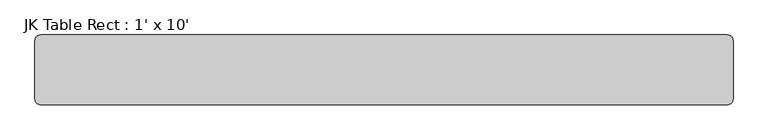
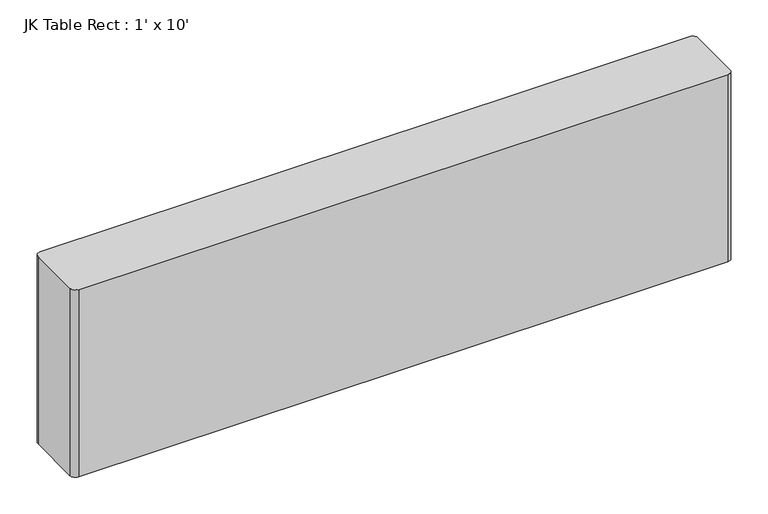
"""IFC4 building model written with IfcOpenShell, lengths in millimetres: furniture geometry, JK Table Rect : 1' x 10'."""

import ifcopenshell
import ifcopenshell.guid

model = None  # the IFC model being written
_history = None  # IfcOwnerHistory: only IFC2X3 demands one
_inside = {}  # id of a spatial element -> (the spatial element, [elements in it])
_under = {}  # id of a project, library or spatial element -> (it, [spatial elements below it])
_declared = {}  # id of a project -> (the project, [libraries it declares])
_typed = {}  # id of a type object -> (the type object, [elements of that type])
_made_of = {}  # id of a material, layer set ... -> (it, [elements and type objects made of it])


def new_model(schema):
    """Start an empty IFC model of exactly this schema.

    Asked for "IFC4X3", IfcOpenShell would pick the latest addendum, in which some entities
    have other attributes; the version numbers below select the first issue.
    IFC2X3 requires an IfcOwnerHistory on every rooted entity: one is made here for all.
    """
    global model, _history
    if schema == "IFC4X3":
        model = ifcopenshell.file(schema_version=(4, 3, 0, 0))
    else:
        model = ifcopenshell.file(schema=schema)
    _inside.clear()
    _under.clear()
    _declared.clear()
    _typed.clear()
    _made_of.clear()
    _history = None
    if model.schema == "IFC2X3":
        org = make("IfcOrganization", Name="unknown")
        user = make(
            "IfcPersonAndOrganization",
            ThePerson=make("IfcPerson", FamilyName="unknown"),
            TheOrganization=org,
        )
        app = make(
            "IfcApplication",
            ApplicationDeveloper=org,
            Version="unknown",
            ApplicationFullName="unknown",
            ApplicationIdentifier="unknown",
        )
        _history = make(
            "IfcOwnerHistory",
            OwningUser=user,
            OwningApplication=app,
            ChangeAction="ADDED",
            CreationDate=0,
        )
    return model


def make(cls, **values):
    """One entity of the class cls with the attributes given. An attribute that is None is left unset."""
    return model.create_entity(
        cls, **{name: value for name, value in values.items() if value is not None}
    )


def rooted(cls, **values):
    """An entity with a GlobalId (a new one), such as an element, a storey or a relation."""
    return make(cls, GlobalId=ifcopenshell.guid.new(), OwnerHistory=_history, **values)


def si_unit(unit_type, name, prefix=None):
    """IfcSIUnit, for example si_unit("LENGTHUNIT", "METRE", prefix="MILLI")."""
    return make("IfcSIUnit", UnitType=unit_type, Prefix=prefix, Name=name)


def assignment(units):
    """IfcUnitAssignment: the units of a project."""
    return None if units is None else make("IfcUnitAssignment", Units=units)


def point(xyz):
    """IfcCartesianPoint."""
    return None if xyz is None else make("IfcCartesianPoint", Coordinates=xyz)


def direction(xyz):
    """IfcDirection."""
    return None if xyz is None else make("IfcDirection", DirectionRatios=xyz)


def frame(location, z_axis=None, x_axis=None):
    """IfcAxis2Placement3D, a coordinate frame: its origin and axes. An axis left out is left unset."""
    return make(
        "IfcAxis2Placement3D",
        Location=point(location),
        Axis=direction(z_axis),
        RefDirection=direction(x_axis),
    )


def frame_2d(location, x_axis=None):
    """IfcAxis2Placement2D, a coordinate frame in the plane: its origin and x axis."""
    return make(
        "IfcAxis2Placement2D", Location=point(location), RefDirection=direction(x_axis)
    )


def origin():
    """The frame at (0, 0, 0) with its axes left unset."""
    return frame((0.0, 0.0, 0.0))


def origin_with_axes():
    """The frame at (0, 0, 0) with the z axis (0, 0, 1) and the x axis (1, 0, 0) written out."""
    return frame((0.0, 0.0, 0.0), z_axis=(0.0, 0.0, 1.0), x_axis=(1.0, 0.0, 0.0))


def place(relative_to, where):
    """IfcLocalPlacement: puts the frame where relative to a parent placement (None: the world)."""
    return make(
        "IfcLocalPlacement", PlacementRelTo=relative_to, RelativePlacement=where
    )


def context(
    kind, dimensions, precision=None, world=None, true_north=None, identifier=None
):
    """IfcGeometricRepresentationContext, for example the 3D "Model" context."""
    return make(
        "IfcGeometricRepresentationContext",
        ContextIdentifier=identifier,
        ContextType=kind,
        CoordinateSpaceDimension=dimensions,
        Precision=precision,
        WorldCoordinateSystem=world,
        TrueNorth=true_north,
    )


def project(units=None, contexts=None):
    """IfcProject with its units and contexts."""
    return rooted(
        "IfcProject",
        Name="project",
        RepresentationContexts=contexts,
        UnitsInContext=assignment(units),
    )


def spatial(cls, under=None, at=None, **own):
    """A site, building, storey or space (cls), placed at a placement, below another one or the project."""
    s = rooted(cls, ObjectPlacement=at, **own)
    if under is not None:
        _under.setdefault(under.id(), (under, []))[1].append(s)
    return s


def polyline(points):
    """IfcPolyline through the points."""
    return make("IfcPolyline", Points=[point(p) for p in points])


def circle_curve(where, radius):
    """IfcCircle in the frame where."""
    return make("IfcCircle", Position=where, Radius=radius)


def trimmed(basis, trim1, trim2, sense, master):
    """IfcTrimmedCurve: the piece of a basis curve between two trims."""
    return make(
        "IfcTrimmedCurve",
        BasisCurve=basis,
        Trim1=trim1,
        Trim2=trim2,
        SenseAgreement=sense,
        MasterRepresentation=master,
    )


def segment(curve, same_sense, transition):
    """IfcCompositeCurveSegment."""
    return make(
        "IfcCompositeCurveSegment",
        Transition=transition,
        SameSense=same_sense,
        ParentCurve=curve,
    )


def composite_curve(segments, self_intersect=None):
    """IfcCompositeCurve: segments joined end to end."""
    return make("IfcCompositeCurve", Segments=segments, SelfIntersect=self_intersect)


def outline(outer, holes=None, kind="AREA"):
    """IfcArbitraryClosedProfileDef: a profile drawn as a closed curve; with holes, ...WithVoids."""
    if holes is None:
        return make("IfcArbitraryClosedProfileDef", ProfileType=kind, OuterCurve=outer)
    return make(
        "IfcArbitraryProfileDefWithVoids",
        ProfileType=kind,
        OuterCurve=outer,
        InnerCurves=holes,
    )


def extrude(swept, where, along, depth):
    """IfcExtrudedAreaSolid: the profile swept, set in the frame where, extruded along a direction by depth."""
    return make(
        "IfcExtrudedAreaSolid",
        SweptArea=swept,
        Position=where,
        ExtrudedDirection=direction(along),
        Depth=depth,
    )


def shape(context_of_items, identifier, shape_type, items):
    """IfcShapeRepresentation: the items that make up one representation, for example the "Body"."""
    return make(
        "IfcShapeRepresentation",
        ContextOfItems=context_of_items,
        RepresentationIdentifier=identifier,
        RepresentationType=shape_type,
        Items=items,
    )


def source(mapping_origin, context_of_items, identifier, shape_type, items):
    """IfcRepresentationMap: a shape defined once, which mapped items show again and again."""
    return make(
        "IfcRepresentationMap",
        MappingOrigin=mapping_origin,
        MappedRepresentation=shape(context_of_items, identifier, shape_type, items),
    )


def transform(
    local_origin,
    x_axis=None,
    y_axis=None,
    z_axis=None,
    scale=None,
    scale2=None,
    scale3=None,
    uniform=True,
):
    """IfcCartesianTransformationOperator3D, or its non-uniform kind. x_axis, y_axis, z_axis: its Axis1, 2, 3."""
    if uniform:
        return make(
            "IfcCartesianTransformationOperator3D",
            Axis1=direction(x_axis),
            Axis2=direction(y_axis),
            LocalOrigin=point(local_origin),
            Scale=scale,
            Axis3=direction(z_axis),
        )
    return make(
        "IfcCartesianTransformationOperator3DnonUniform",
        Axis1=direction(x_axis),
        Axis2=direction(y_axis),
        LocalOrigin=point(local_origin),
        Scale=scale,
        Axis3=direction(z_axis),
        Scale2=scale2,
        Scale3=scale3,
    )


def mapped(mapping_source, mapping_target):
    """IfcMappedItem: shows the shape of a source again, moved by a transform."""
    return make(
        "IfcMappedItem", MappingSource=mapping_source, MappingTarget=mapping_target
    )


def made_of(thing, what):
    """Note that an element or type object is made of a material, layer set ...; save() writes the relation."""
    if what is not None:
        _made_of.setdefault(what.id(), (what, []))[1].append(thing)
    return thing


def element(
    cls,
    number,
    at=None,
    inside=None,
    cuts=None,
    type_object=None,
    material=None,
    context=None,
    identifier="Body",
    shape_type=None,
    held_by="IfcProductDefinitionShape",
    body=None,
    shapes=None,
    **own,
):
    """One element of the class cls, such as IfcWall. Its Tag is "e" and its number.

    at: its placement. inside: the storey or other place that contains it. cuts: it is an
    opening in that element (IfcRelVoidsElement). A single representation is given by context,
    identifier, shape_type and body (its items); several are given by shapes. held_by: the class
    of the entity that holds the representations. save() writes the other relations.
    """
    e = rooted(cls, Tag="e%d" % number, ObjectPlacement=at, **own)
    if body is not None:
        shapes = [shape(context, identifier, shape_type, body)]
    if shapes is not None:
        e.Representation = make(held_by, Representations=shapes)
    if inside is not None:
        _inside.setdefault(inside.id(), (inside, []))[1].append(e)
    if cuts is not None:
        rooted(
            "IfcRelVoidsElement", RelatingBuildingElement=cuts, RelatedOpeningElement=e
        )
    if type_object is not None:
        _typed.setdefault(type_object.id(), (type_object, []))[1].append(e)
    return made_of(e, material)


def aggregate(whole, parts):
    """IfcRelAggregates: a whole, such as a stair, and the parts it consists of."""
    return rooted("IfcRelAggregates", RelatingObject=whole, RelatedObjects=parts)


def save(model, path):
    """Write the relations noted so far, then the file.

    IfcRelAggregates (storeys below a building ...), IfcRelContainedInSpatialStructure (elements
    in a storey), IfcRelDefinesByType, IfcRelAssociatesMaterial and IfcRelDeclares: one each for
    every whole, place, type object, material and project.
    """
    for whole, parts in _under.values():
        aggregate(whole, parts)
    for where, things in _inside.values():
        rooted(
            "IfcRelContainedInSpatialStructure",
            RelatedElements=things,
            RelatingStructure=where,
        )
    for kind, things in _typed.values():
        rooted("IfcRelDefinesByType", RelatedObjects=things, RelatingType=kind)
    for what, things in _made_of.values():
        rooted("IfcRelAssociatesMaterial", RelatedObjects=things, RelatingMaterial=what)
    for by, libraries in _declared.values():
        rooted("IfcRelDeclares", RelatingContext=by, RelatedDefinitions=libraries)
    model.write(path)


def jk_table_rect_1_x_10_fe09fb00(model_context):
    return source(origin(), model_context, "Body", "SweptSolid", [
        extrude(outline(composite_curve([segment(trimmed(circle_curve(frame_2d((1436.6573665, 160.5455296)), 25.4), [point((1436.6573665, 185.9455296))], [point((1462.0573665, 160.5455296))], False, "CARTESIAN"), True, "CONTINUOUS"), segment(polyline([(1462.0573665, 160.5455296), (1462.0573665, -93.4544704)]), True, "CONTINUOUS"), segment(trimmed(circle_curve(frame_2d((1436.6573665, -93.4544704)), 25.4), [point((1462.0573665, -93.4544704))], [point((1436.6573665, -118.8544704))], False, "CARTESIAN"), True, "CONTINUOUS"), segment(polyline([(1436.6573665, -118.8544704), (-1560.5426335, -118.8544704)]), True, "CONTINUOUS"), segment(trimmed(circle_curve(frame_2d((-1560.5426335, -93.4544704)), 25.4), [point((-1560.5426335, -118.8544704))], [point((-1585.9426335, -93.4544704))], False, "CARTESIAN"), True, "CONTINUOUS"), segment(polyline([(-1585.9426335, -93.4544704), (-1585.9426335, 160.5455296)]), True, "CONTINUOUS"), segment(trimmed(circle_curve(frame_2d((-1560.5426335, 160.5455296)), 25.4), [point((-1585.9426335, 160.5455296))], [point((-1560.5426335, 185.9455296))], False, "CARTESIAN"), True, "CONTINUOUS"), segment(polyline([(-1560.5426335, 185.9455296), (1436.6573665, 185.9455296)]), True, "CONTINUOUS")], self_intersect=False)), origin_with_axes(), (0.0, 0.0, 1.0), 914.4),
    ])


if __name__ == "__main__":
    model = new_model("IFC4")
    model_context = context("Model", 3, world=origin())
    ifc_project = project(units=[si_unit("LENGTHUNIT", "METRE", prefix="MILLI")], contexts=[model_context])
    site = spatial("IfcSite", under=ifc_project)
    building = spatial("IfcBuilding", under=site)
    placement = place(None, origin())
    jk_table_rect_1_x_10_shape = jk_table_rect_1_x_10_fe09fb00(model_context)
    element("IfcFurniture", 1, ObjectType="JK Table Rect : 1' x 10'", at=placement, inside=building, context=model_context, shape_type="MappedRepresentation", body=[
        mapped(jk_table_rect_1_x_10_shape, transform((0.0, 0.0, 0.0), x_axis=(1.0, 0.0, 0.0), y_axis=(0.0, 1.0, 0.0), z_axis=(0.0, 0.0, 1.0))),
    ])
    save(model, "model.ifc")

# Revit data of these elements
# Type "JK Table Rect : 1' x 10'"
#   Width = 10' - 0"
#   Height = 3' - 0"
#   Depth = 1' - 0"
#   Corner Radius = 0' - 1"
#   Status [instance default] = none
#   Default Elevation = 0
